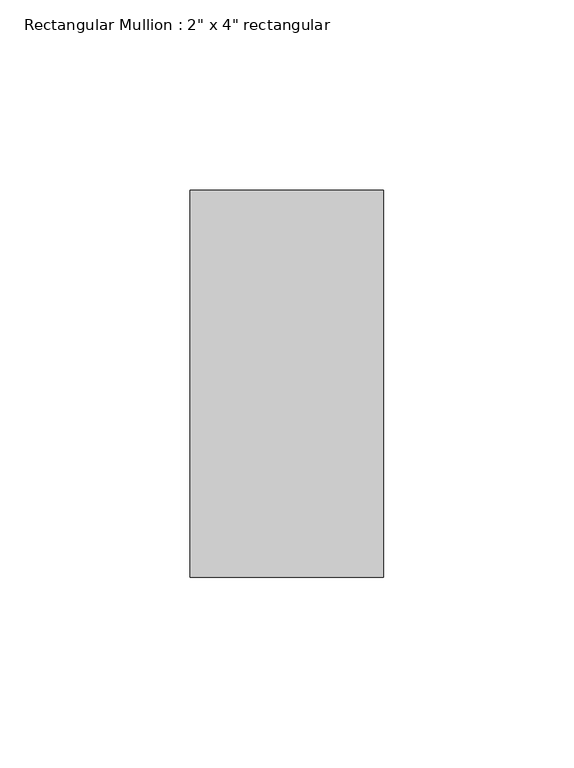
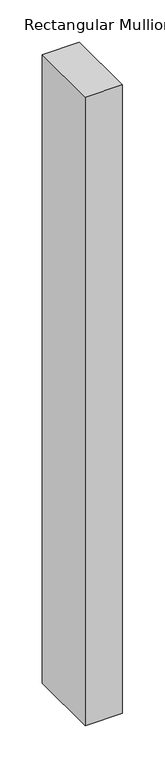
"""IFC4 building model written with IfcOpenShell, lengths in millimetres: member geometry."""

import ifcopenshell
import ifcopenshell.guid

model = None  # the IFC model being written
_history = None  # IfcOwnerHistory: only IFC2X3 demands one
_inside = {}  # id of a spatial element -> (the spatial element, [elements in it])
_under = {}  # id of a project, library or spatial element -> (it, [spatial elements below it])
_declared = {}  # id of a project -> (the project, [libraries it declares])
_typed = {}  # id of a type object -> (the type object, [elements of that type])
_made_of = {}  # id of a material, layer set ... -> (it, [elements and type objects made of it])


def new_model(schema):
    """Start an empty IFC model of exactly this schema.

    Asked for "IFC4X3", IfcOpenShell would pick the latest addendum, in which some entities
    have other attributes; the version numbers below select the first issue.
    IFC2X3 requires an IfcOwnerHistory on every rooted entity: one is made here for all.
    """
    global model, _history
    if schema == "IFC4X3":
        model = ifcopenshell.file(schema_version=(4, 3, 0, 0))
    else:
        model = ifcopenshell.file(schema=schema)
    _inside.clear()
    _under.clear()
    _declared.clear()
    _typed.clear()
    _made_of.clear()
    _history = None
    if model.schema == "IFC2X3":
        org = make("IfcOrganization", Name="unknown")
        user = make(
            "IfcPersonAndOrganization",
            ThePerson=make("IfcPerson", FamilyName="unknown"),
            TheOrganization=org,
        )
        app = make(
            "IfcApplication",
            ApplicationDeveloper=org,
            Version="unknown",
            ApplicationFullName="unknown",
            ApplicationIdentifier="unknown",
        )
        _history = make(
            "IfcOwnerHistory",
            OwningUser=user,
            OwningApplication=app,
            ChangeAction="ADDED",
            CreationDate=0,
        )
    return model


def make(cls, **values):
    """One entity of the class cls with the attributes given. An attribute that is None is left unset."""
    return model.create_entity(
        cls, **{name: value for name, value in values.items() if value is not None}
    )


def rooted(cls, **values):
    """An entity with a GlobalId (a new one), such as an element, a storey or a relation."""
    return make(cls, GlobalId=ifcopenshell.guid.new(), OwnerHistory=_history, **values)


def si_unit(unit_type, name, prefix=None):
    """IfcSIUnit, for example si_unit("LENGTHUNIT", "METRE", prefix="MILLI")."""
    return make("IfcSIUnit", UnitType=unit_type, Prefix=prefix, Name=name)


def assignment(units):
    """IfcUnitAssignment: the units of a project."""
    return None if units is None else make("IfcUnitAssignment", Units=units)


def point(xyz):
    """IfcCartesianPoint."""
    return None if xyz is None else make("IfcCartesianPoint", Coordinates=xyz)


def direction(xyz):
    """IfcDirection."""
    return None if xyz is None else make("IfcDirection", DirectionRatios=xyz)


def frame(location, z_axis=None, x_axis=None):
    """IfcAxis2Placement3D, a coordinate frame: its origin and axes. An axis left out is left unset."""
    return make(
        "IfcAxis2Placement3D",
        Location=point(location),
        Axis=direction(z_axis),
        RefDirection=direction(x_axis),
    )


def origin():
    """The frame at (0, 0, 0) with its axes left unset."""
    return frame((0.0, 0.0, 0.0))


def place(relative_to, where):
    """IfcLocalPlacement: puts the frame where relative to a parent placement (None: the world)."""
    return make(
        "IfcLocalPlacement", PlacementRelTo=relative_to, RelativePlacement=where
    )


def context(
    kind, dimensions, precision=None, world=None, true_north=None, identifier=None
):
    """IfcGeometricRepresentationContext, for example the 3D "Model" context."""
    return make(
        "IfcGeometricRepresentationContext",
        ContextIdentifier=identifier,
        ContextType=kind,
        CoordinateSpaceDimension=dimensions,
        Precision=precision,
        WorldCoordinateSystem=world,
        TrueNorth=true_north,
    )


def project(units=None, contexts=None):
    """IfcProject with its units and contexts."""
    return rooted(
        "IfcProject",
        Name="project",
        RepresentationContexts=contexts,
        UnitsInContext=assignment(units),
    )


def spatial(cls, under=None, at=None, **own):
    """A site, building, storey or space (cls), placed at a placement, below another one or the project."""
    s = rooted(cls, ObjectPlacement=at, **own)
    if under is not None:
        _under.setdefault(under.id(), (under, []))[1].append(s)
    return s


def polyline(points):
    """IfcPolyline through the points."""
    return make("IfcPolyline", Points=[point(p) for p in points])


def outline(outer, holes=None, kind="AREA"):
    """IfcArbitraryClosedProfileDef: a profile drawn as a closed curve; with holes, ...WithVoids."""
    if holes is None:
        return make("IfcArbitraryClosedProfileDef", ProfileType=kind, OuterCurve=outer)
    return make(
        "IfcArbitraryProfileDefWithVoids",
        ProfileType=kind,
        OuterCurve=outer,
        InnerCurves=holes,
    )


def extrude(swept, where, along, depth):
    """IfcExtrudedAreaSolid: the profile swept, set in the frame where, extruded along a direction by depth."""
    return make(
        "IfcExtrudedAreaSolid",
        SweptArea=swept,
        Position=where,
        ExtrudedDirection=direction(along),
        Depth=depth,
    )


def shape(context_of_items, identifier, shape_type, items):
    """IfcShapeRepresentation: the items that make up one representation, for example the "Body"."""
    return make(
        "IfcShapeRepresentation",
        ContextOfItems=context_of_items,
        RepresentationIdentifier=identifier,
        RepresentationType=shape_type,
        Items=items,
    )


def source(mapping_origin, context_of_items, identifier, shape_type, items):
    """IfcRepresentationMap: a shape defined once, which mapped items show again and again."""
    return make(
        "IfcRepresentationMap",
        MappingOrigin=mapping_origin,
        MappedRepresentation=shape(context_of_items, identifier, shape_type, items),
    )


def transform(
    local_origin,
    x_axis=None,
    y_axis=None,
    z_axis=None,
    scale=None,
    scale2=None,
    scale3=None,
    uniform=True,
):
    """IfcCartesianTransformationOperator3D, or its non-uniform kind. x_axis, y_axis, z_axis: its Axis1, 2, 3."""
    if uniform:
        return make(
            "IfcCartesianTransformationOperator3D",
            Axis1=direction(x_axis),
            Axis2=direction(y_axis),
            LocalOrigin=point(local_origin),
            Scale=scale,
            Axis3=direction(z_axis),
        )
    return make(
        "IfcCartesianTransformationOperator3DnonUniform",
        Axis1=direction(x_axis),
        Axis2=direction(y_axis),
        LocalOrigin=point(local_origin),
        Scale=scale,
        Axis3=direction(z_axis),
        Scale2=scale2,
        Scale3=scale3,
    )


def mapped(mapping_source, mapping_target):
    """IfcMappedItem: shows the shape of a source again, moved by a transform."""
    return make(
        "IfcMappedItem", MappingSource=mapping_source, MappingTarget=mapping_target
    )


def made_of(thing, what):
    """Note that an element or type object is made of a material, layer set ...; save() writes the relation."""
    if what is not None:
        _made_of.setdefault(what.id(), (what, []))[1].append(thing)
    return thing


def element(
    cls,
    number,
    at=None,
    inside=None,
    cuts=None,
    type_object=None,
    material=None,
    context=None,
    identifier="Body",
    shape_type=None,
    held_by="IfcProductDefinitionShape",
    body=None,
    shapes=None,
    **own,
):
    """One element of the class cls, such as IfcWall. Its Tag is "e" and its number.

    at: its placement. inside: the storey or other place that contains it. cuts: it is an
    opening in that element (IfcRelVoidsElement). A single representation is given by context,
    identifier, shape_type and body (its items); several are given by shapes. held_by: the class
    of the entity that holds the representations. save() writes the other relations.
    """
    e = rooted(cls, Tag="e%d" % number, ObjectPlacement=at, **own)
    if body is not None:
        shapes = [shape(context, identifier, shape_type, body)]
    if shapes is not None:
        e.Representation = make(held_by, Representations=shapes)
    if inside is not None:
        _inside.setdefault(inside.id(), (inside, []))[1].append(e)
    if cuts is not None:
        rooted(
            "IfcRelVoidsElement", RelatingBuildingElement=cuts, RelatedOpeningElement=e
        )
    if type_object is not None:
        _typed.setdefault(type_object.id(), (type_object, []))[1].append(e)
    return made_of(e, material)


def aggregate(whole, parts):
    """IfcRelAggregates: a whole, such as a stair, and the parts it consists of."""
    return rooted("IfcRelAggregates", RelatingObject=whole, RelatedObjects=parts)


def save(model, path):
    """Write the relations noted so far, then the file.

    IfcRelAggregates (storeys below a building ...), IfcRelContainedInSpatialStructure (elements
    in a storey), IfcRelDefinesByType, IfcRelAssociatesMaterial and IfcRelDeclares: one each for
    every whole, place, type object, material and project.
    """
    for whole, parts in _under.values():
        aggregate(whole, parts)
    for where, things in _inside.values():
        rooted(
            "IfcRelContainedInSpatialStructure",
            RelatedElements=things,
            RelatingStructure=where,
        )
    for kind, things in _typed.values():
        rooted("IfcRelDefinesByType", RelatedObjects=things, RelatingType=kind)
    for what, things in _made_of.values():
        rooted("IfcRelAssociatesMaterial", RelatedObjects=things, RelatingMaterial=what)
    for by, libraries in _declared.values():
        rooted("IfcRelDeclares", RelatingContext=by, RelatedDefinitions=libraries)
    model.write(path)


def member_498deac5(model_context):
    return source(origin(), model_context, "Body", "SweptSolid", [
        extrude(outline(polyline([(0.0, 50.8), (0.0, -50.8), (-50.8, -50.8), (-50.8, 50.8), (0.0, 50.8)])), frame((0.0, 0.0, -907.1428571), z_axis=(0.0, 0.0, 1.0), x_axis=(1.0, 0.0, 0.0)), (0.0, 0.0, 1.0), 907.1428571),
    ])


if __name__ == "__main__":
    model = new_model("IFC4")
    model_context = context("Model", 3, world=origin())
    ifc_project = project(units=[si_unit("LENGTHUNIT", "METRE", prefix="MILLI")], contexts=[model_context])
    site = spatial("IfcSite", under=ifc_project)
    building = spatial("IfcBuilding", under=site)
    placement = place(None, origin())
    member_shape = member_498deac5(model_context)
    element("IfcMember", 1, ObjectType="Rectangular Mullion : 2\" x 4\" rectangular", at=placement, inside=building, context=model_context, shape_type="MappedRepresentation", body=[
        mapped(member_shape, transform((0.0, 0.0, 0.0), x_axis=(1.0, 0.0, 0.0), y_axis=(0.0, 1.0, 0.0), z_axis=(0.0, 0.0, 1.0))),
    ])
    save(model, "model.ifc")

# Revit data of these elements
# Type "Rectangular Mullion : 2\" x 4\" rectangular"
#   built-in parameter 1007304 = 0.333333 (stored number, unit not read)
#   built-in parameter 1007301 = 0.0833333 (stored number, unit not read)
#   built-in parameter 1007300 = 0.0833333 (stored number, unit not read)
